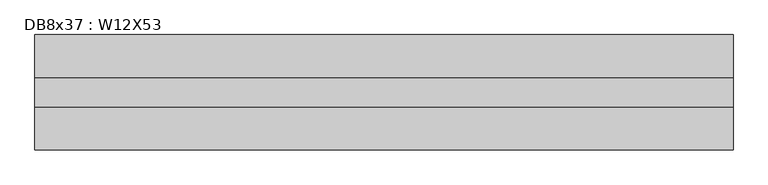
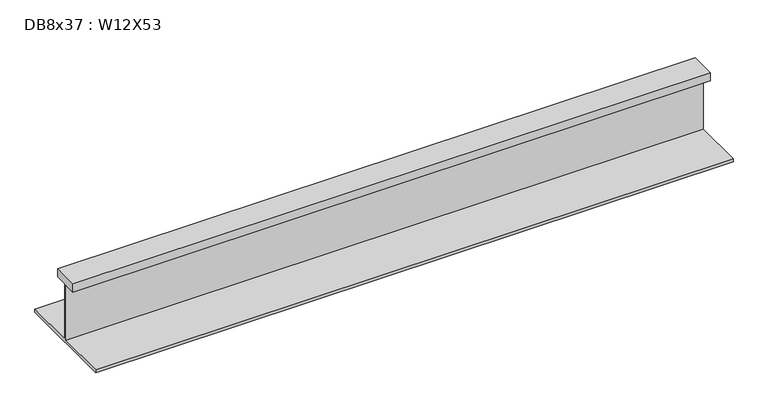
"""IFC4 building model written with IfcOpenShell, lengths in millimetres: beam geometry, DB8x37 : W12X53."""

from ifc_helpers import new_model, si_unit, frame, origin, place, context, project, spatial, polyline, outline, extrude, source, transform, mapped, element, save


def db8x37_w12x53_fa12a80e(model_context):
    return source(origin(), model_context, "Body", "SweptSolid", [
        extrude(outline(polyline([(38.1, 145.415), (38.1, 120.015), (2.921, 120.015), (2.921, -48.4505), (152.4, -48.4505), (152.4, -58.1025), (-152.4, -58.1025), (-152.4, -48.4505), (-2.921, -48.4505), (-2.921, 120.015), (-38.1, 120.015), (-38.1, 145.415), (38.1, 145.415)])), frame((-854.329, 0.0, 0.0), z_axis=(1.0, 0.0, 0.0), x_axis=(0.0, 1.0, 0.0)), (0.0, 0.0, 1.0), 1844.929),
    ])


if __name__ == "__main__":
    model = new_model("IFC4")
    model_context = context("Model", 3, world=origin())
    ifc_project = project(units=[si_unit("LENGTHUNIT", "METRE", prefix="MILLI")], contexts=[model_context])
    site = spatial("IfcSite", under=ifc_project)
    building = spatial("IfcBuilding", under=site)
    placement = place(None, origin())
    db8x37_w12x53_shape = db8x37_w12x53_fa12a80e(model_context)
    element("IfcBeam", 1, ObjectType="DB8x37 : W12X53", at=placement, inside=building, context=model_context, shape_type="MappedRepresentation", body=[
        mapped(db8x37_w12x53_shape, transform((0.0, 0.0, 0.0), x_axis=(1.0, 0.0, 0.0), y_axis=(0.0, 1.0, 0.0), z_axis=(0.0, 0.0, 1.0))),
    ])
    save(model, "model.ifc")

# Revit data of these elements
# Type "DB8x37 : W12X53"
#   Assembly Code = "B10"
#   W = 53
#   Length [instance default] = 5' - 0"
#   bf = 0' - 10"
#   d = 1' - 0.1"
#   k = 0' - 1 3/8"
#   k2 = 0' - 0.8"
#   tf = 0' - 0.575"
#   tw = 0' - 0.345"
#   A = 0.108333 SF
#   Structural Material [instance default] = Steel ASTM A992
# Element 1 (IfcBeam, "DB8x37 : W12X53")
#   Materials on its faces: "Steel ASTM A992"
# Materials
#   "Steel ASTM A992": class "Metal", colour RGB 199 199 199, transparency 0, Description = "Structural steel 50ksi", Cost = 0
